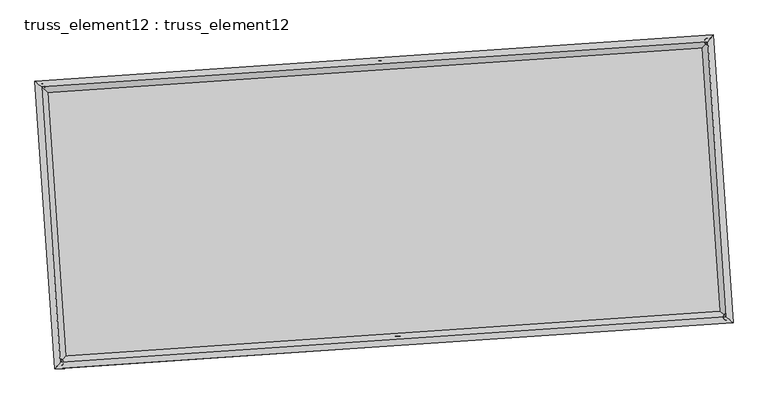
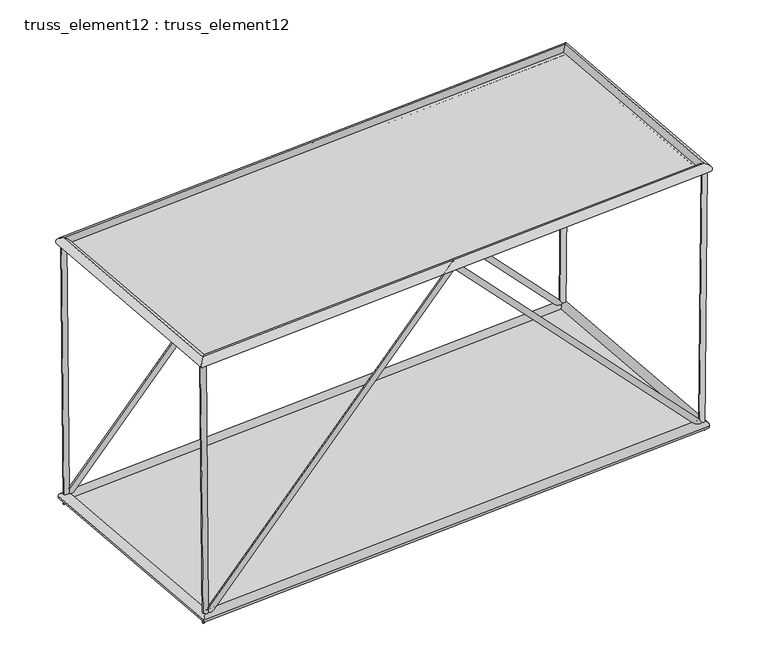
"""IFC4 building model written with IfcOpenShell, lengths in millimetres: plate geometry, truss_element12 : truss_element12."""

from ifc_helpers import new_model, si_unit, frame, origin, origin_with_axes, place, context, project, spatial, polyline, circle_curve, ellipse_curve, outline, extrude, source, transform, mapped, element, save
from ifc_brep_helpers import plane_surface, cylinder_surface, advanced_brep


def truss_element12_truss_element12_3d995396(model_context):
    return source(origin(), model_context, "Body", "SolidModel", [
        advanced_brep(
        [(-3712.6408018, 2272.9715483, 5000.2484753), (-3811.7396164, 2259.6106092, 4999.2944024), (-3666.1125982, 2276.1441296, 122.9707334), (-3762.8742846, 2262.9425505, -122.9707334), (1064.1401196, 2598.6820811, 5071.8896086), (1064.5820396, 2592.1084463, 4927.6451952), (5793.5718475, 2921.1640524, 122.9648431), (5891.1891295, 2921.2164361, -122.9648431), (5840.9148394, 2924.392191, 5000.2487538), (5940.9098971, 2924.6067063, 4999.2779762)],
        [
            (0, 1, circle_curve(frame((-3762.1902091, 2266.2910788, 4999.7714389), z_axis=(-0.009539353531426898, -0.0006504522548332356, 0.9999542877782298), x_axis=(-0.13360948886072543, 0.9910338579689815, -0.0006299567385858392)), 50.0)),
            (1, 0, circle_curve(frame((-3762.1902091, 2266.2910788, 4999.7714389), z_axis=(-0.009539353531426898, -0.0006504522548332356, 0.9999542877782298), x_axis=(-0.13360948886072543, 0.9910338579689815, -0.0006299567385858392)), 50.0)),
            (0, 2),
            (2, 3, ellipse_curve(frame((-3714.4934414, 2269.54334, 0.0), z_axis=(-0.9275444537546121, -0.06324573037496291, 0.368322228352289), x_axis=(0.3674689716323781, 0.02505631229527238, 0.9296981962452139)), 132.5575344, 50.0)),
            (3, 1),
            (3, 2, ellipse_curve(frame((-3714.4934414, 2269.54334, 0.0), z_axis=(-0.9275444537546121, -0.06324573037496291, 0.368322228352289), x_axis=(0.3674689716323781, 0.02505631229527238, 0.9296981962452139)), 132.5575344, 50.0)),
            (2, 4),
            (4, 5, ellipse_curve(frame((1064.3610796, 2595.3952637, 4999.7674019), z_axis=(-0.9976833951243609, -0.06802823816388774, 4.365141464773057e-05), x_axis=(-4.355029160929896e-05, -2.969528831717673e-06, -0.9999999990472769)), 72.279252, 50.0)),
            (5, 3),
            (5, 4, ellipse_curve(frame((1064.3610796, 2595.3952637, 4999.7674019), z_axis=(-0.9976833951243609, -0.06802823816388774, 4.365141464773057e-05), x_axis=(-4.355029160929896e-05, -2.969528831717673e-06, -0.9999999990472769)), 72.279252, 50.0)),
            (4, 6),
            (6, 7, ellipse_curve(frame((5842.3804885, 2921.1902443, 0.0), z_axis=(-0.9275912472386779, -0.06324892104476065, -0.36820381860169205), x_axis=(-0.36735083619027376, -0.02504825708855556, 0.9297450983829559)), 132.5444982, 50.0)),
            (7, 5),
            (7, 6, ellipse_curve(frame((5842.3804885, 2921.1902443, 0.0), z_axis=(-0.9275912472386779, -0.06324892104476065, -0.36820381860169205), x_axis=(-0.36735083619027376, -0.02504825708855556, 0.9297450983829559)), 132.5444982, 50.0)),
            (8, 9, circle_curve(frame((5890.9123683, 2924.4994486, 4999.763365), z_axis=(0.009706375954598431, 0.0006618408789518583, 0.999952672996317), x_axis=(-0.0021514761027001668, 0.999997480140261, -0.0006409865112665113)), 50.0)),
            (9, 8, circle_curve(frame((5890.9123683, 2924.4994486, 4999.763365), z_axis=(0.009706375954598431, 0.0006618408789518583, 0.999952672996317), x_axis=(-0.0021514761027001668, 0.999997480140261, -0.0006409865112665113)), 50.0)),
            (6, 8),
            (9, 7),
        ],
        [
            plane_surface(frame((-3762.1902091, 2316.2910682, 4999.803963), z_axis=(-0.009539353531428214, -0.0006504522548355754, 0.9999542877782297), x_axis=(0.9999544993319458, -6.205176354079358e-06, 0.009539351513250697))),
            cylinder_surface(frame((-3762.1902091, 2266.2910788, 4999.7714389), z_axis=(-0.009539353531426898, -0.0006504522548332356, 0.9999542877782298), x_axis=(-0.13360948886072543, 0.9910338579689815, -0.0006299567385858392)), 50.0),
            cylinder_surface(frame((-3714.4934414, 2269.54334, 0.0), z_axis=(-0.6901903584114236, -0.0470614568808942, -0.7220958997475049), x_axis=(-0.020415575362847597, 0.998752120640053, -0.04557856732721049)), 50.0),
            cylinder_surface(frame((1064.3610796, 2595.3952637, 4999.7674019), z_axis=(-0.6901274608072349, -0.047057168132365004, 0.7221562924790736), x_axis=(-0.11534925319653908, 0.9922789540252682, -0.04557441371559841)), 50.0),
            plane_surface(frame((5890.9123683, 2874.4994596, 4999.7964586), z_axis=(0.009706375954601498, 0.0006618408789477092, 0.9999526729963171), x_axis=(0.9999528920233334, -6.42437903231041e-06, -0.009706373828542777))),
            cylinder_surface(frame((5842.3804885, 2921.1902443, 0.0), z_axis=(-0.00970637595459843, -0.0006618408789518581, -0.9999526729963167), x_axis=(-0.0021514761027001668, 0.999997480140261, -0.0006409865112665113)), 50.0),
        ],
        [
            (0, [[1, 2]]),
            (1, [[-1, 3, 4, 5]]),
            (1, [[-2, -5, 6, -3]]),
            (2, [[-4, 7, 8, 9]]),
            (2, [[-6, -9, 10, -7]]),
            (3, [[-8, 11, 12, 13]]),
            (3, [[-10, -13, 14, -11]]),
            (4, [[15, 16]]),
            (5, [[-12, 17, -16, 18]]),
            (5, [[-14, -18, -15, -17]]),
        ],
    ),
        advanced_brep(
        [(-3440.5278489, -1717.762036, 5000.2484753), (-3539.6266635, -1731.1229751, 4999.2944024), (-3393.9996453, -1714.5894547, 122.9707334), (-3490.7613317, -1727.7910338, -122.9707334), (1336.2530725, -1392.0515032, 5071.8896086), (1336.6949926, -1398.625138, 4927.6451952), (6065.6848004, -1069.5695319, 122.9648431), (6163.3020824, -1069.5171482, -122.9648431), (6113.0277923, -1066.3413933, 5000.2487538), (6213.0228501, -1066.126878, 4999.2779762)],
        [
            (0, 1, circle_curve(frame((-3490.0772562, -1724.4425055, 4999.7714389), z_axis=(-0.009539353531426684, -0.0006504522548331923, 0.9999542877782298), x_axis=(-0.1336094888607254, 0.9910338579689815, -0.0006299567385858533)), 50.0)),
            (1, 0, circle_curve(frame((-3490.0772562, -1724.4425055, 4999.7714389), z_axis=(-0.009539353531426684, -0.0006504522548331923, 0.9999542877782298), x_axis=(-0.1336094888607254, 0.9910338579689815, -0.0006299567385858533)), 50.0)),
            (0, 2),
            (2, 3, ellipse_curve(frame((-3442.3804885, -1721.1902443, 0.0), z_axis=(-0.9275444537546114, -0.06324573037496278, 0.3683222283522907), x_axis=(0.36746897163237974, 0.025056312295272495, 0.9296981962452131)), 132.5575344, 50.0)),
            (3, 1),
            (3, 2, ellipse_curve(frame((-3442.3804885, -1721.1902443, 0.0), z_axis=(-0.9275444537546114, -0.06324573037496278, 0.3683222283522907), x_axis=(0.36746897163237974, 0.025056312295272495, 0.9296981962452131)), 132.5575344, 50.0)),
            (2, 4),
            (4, 5, ellipse_curve(frame((1336.4740325, -1395.3383206, 4999.7674019), z_axis=(-0.9976833951243609, -0.06802823816388762, 4.365141464997738e-05), x_axis=(-4.355029161160519e-05, -2.9695288319579026e-06, -0.9999999990472771)), 72.279252, 50.0)),
            (5, 3),
            (5, 4, ellipse_curve(frame((1336.4740325, -1395.3383206, 4999.7674019), z_axis=(-0.9976833951243609, -0.06802823816388762, 4.365141464997738e-05), x_axis=(-4.355029161160519e-05, -2.9695288319579026e-06, -0.9999999990472771)), 72.279252, 50.0)),
            (4, 6),
            (6, 7, ellipse_curve(frame((6114.4934414, -1069.54334, 0.0), z_axis=(-0.927591247238678, -0.06324892104476053, -0.3682038186016914), x_axis=(-0.3673508361902732, -0.025048257088555438, 0.929745098382956)), 132.5444982, 50.0)),
            (7, 5),
            (7, 6, ellipse_curve(frame((6114.4934414, -1069.54334, 0.0), z_axis=(-0.927591247238678, -0.06324892104476053, -0.3682038186016914), x_axis=(-0.3673508361902732, -0.025048257088555438, 0.929745098382956)), 132.5444982, 50.0)),
            (8, 9, circle_curve(frame((6163.0253212, -1066.2341357, 4999.763365), z_axis=(0.009706375954599215, 0.0006618408789519453, 0.999952672996317), x_axis=(-0.002151476102700382, 0.9999974801402611, -0.0006409865112665946)), 50.0)),
            (9, 8, circle_curve(frame((6163.0253212, -1066.2341357, 4999.763365), z_axis=(0.009706375954599215, 0.0006618408789519453, 0.999952672996317), x_axis=(-0.002151476102700382, 0.9999974801402611, -0.0006409865112665946)), 50.0)),
            (6, 8),
            (9, 7),
        ],
        [
            plane_surface(frame((-3490.0772562, -1674.4425161, 4999.803963), z_axis=(-0.009539353531428214, -0.0006504522548355842, 0.9999542877782297), x_axis=(0.9999544993319458, -6.205176354079358e-06, 0.009539351513250697))),
            cylinder_surface(frame((-3490.0772562, -1724.4425055, 4999.7714389), z_axis=(-0.009539353531426684, -0.0006504522548331923, 0.9999542877782298), x_axis=(-0.1336094888607254, 0.9910338579689815, -0.0006299567385858533)), 50.0),
            cylinder_surface(frame((-3442.3804885, -1721.1902443, 0.0), z_axis=(-0.6901903584114265, -0.047061456880894366, -0.7220958997475021), x_axis=(-0.020415575362847802, 0.998752120640053, -0.04557856732721061)), 50.0),
            cylinder_surface(frame((1336.4740325, -1395.3383206, 4999.7674019), z_axis=(-0.6901274608072342, -0.047057168132364824, 0.722156292479074), x_axis=(-0.1153492531965389, 0.9922789540252682, -0.04557441371559837)), 50.0),
            plane_surface(frame((6163.0253212, -1116.2341247, 4999.7964586), z_axis=(0.009706375954601498, 0.0006618408789477163, 0.9999526729963171), x_axis=(0.9999528920233334, -6.424379032754499e-06, -0.009706373828542777))),
            cylinder_surface(frame((6114.4934414, -1069.54334, 0.0), z_axis=(-0.009706375954599215, -0.0006618408789519453, -0.999952672996317), x_axis=(-0.002151476102700382, 0.9999974801402611, -0.0006409865112665946)), 50.0),
        ],
        [
            (0, [[1, 2]]),
            (1, [[-1, 3, 4, 5]]),
            (1, [[-2, -5, 6, -3]]),
            (2, [[-4, 7, 8, 9]]),
            (2, [[-6, -9, 10, -7]]),
            (3, [[-8, 11, 12, 13]]),
            (3, [[-10, -13, 14, -11]]),
            (4, [[15, 16]]),
            (5, [[-12, 17, -16, 18]]),
            (5, [[-14, -18, -15, -17]]),
        ],
    ),
        advanced_brep(
        [(-3490.0793814, -1724.444861, 4909.7714389), (-3490.075131, -1724.4401501, 5089.7714389), (-3762.1877838, 2266.2890336, 5089.7714389), (-3762.1926343, 2266.2931239, 4909.7714389), (5890.9103929, 2924.4971034, 5089.763365), (5890.9143436, 2924.5017939, 4909.763365), (6163.0230458, -1066.2320803, 5089.763365), (6163.0275966, -1066.236191, 4909.763365)],
        [
            (0, 1, ellipse_curve(frame((-3490.0772562, -1724.4425055, 4999.7714389), z_axis=(-0.7535719234052061, 0.6573654662781049, 5.900579994198024e-07), x_axis=(-0.6573654662778425, -0.7535719234054348, 5.900580116710992e-07)), 127.2792206, 90.0)),
            (1, 2),
            (2, 3, ellipse_curve(frame((-3762.1902091, 2266.2910788, 4999.7714389), z_axis=(-0.6573654662778421, -0.7535719234054352, 5.900580091387355e-07), x_axis=(0.7535719234052064, -0.6573654662781044, -5.900579968874395e-07)), 127.2792206, 90.0)),
            (3, 0),
            (1, 0, ellipse_curve(frame((-3490.0772562, -1724.4425055, 4999.7714389), z_axis=(-0.7535719234052061, 0.6573654662781049, 5.900579994198024e-07), x_axis=(-0.6573654662778425, -0.7535719234054348, 5.900580116710992e-07)), 127.2792206, 90.0)),
            (3, 2, ellipse_curve(frame((-3762.1902091, 2266.2910788, 4999.7714389), z_axis=(-0.6573654662778421, -0.7535719234054352, 5.900580091387355e-07), x_axis=(0.7535719234052064, -0.6573654662781044, -5.900579968874395e-07)), 127.2792206, 90.0)),
            (2, 4),
            (4, 5, ellipse_curve(frame((5890.9123683, 2924.4994486, 4999.763365), z_axis=(-0.753571923405209, 0.6573654662781013, 5.90058003013114e-07), x_axis=(-0.6573654662778391, -0.7535719234054377, 5.900580030130607e-07)), 127.2792206, 90.0)),
            (5, 3),
            (5, 4, ellipse_curve(frame((5890.9123683, 2924.4994486, 4999.763365), z_axis=(-0.753571923405209, 0.6573654662781013, 5.90058003013114e-07), x_axis=(-0.6573654662778391, -0.7535719234054377, 5.900580030130607e-07)), 127.2792206, 90.0)),
            (4, 6),
            (6, 7, ellipse_curve(frame((6163.0253212, -1066.2341357, 4999.763365), z_axis=(0.6573654662778391, 0.7535719234054377, -5.900580055454242e-07), x_axis=(-0.7535719234052087, 0.6573654662781017, 5.900580055454772e-07)), 127.2792206, 90.0)),
            (7, 5),
            (7, 6, ellipse_curve(frame((6163.0253212, -1066.2341357, 4999.763365), z_axis=(0.6573654662778391, 0.7535719234054377, -5.900580055454242e-07), x_axis=(-0.7535719234052087, 0.6573654662781017, 5.900580055454772e-07)), 127.2792206, 90.0)),
            (6, 1),
            (0, 7),
        ],
        [
            cylinder_surface(frame((-3490.0772562, -1724.4425055, 4999.7714389), z_axis=(0.06802823822868706, -0.9976833960748777, 0.0), x_axis=(-0.9976833957545878, -0.06802823820684771, 2.53390411256576e-05)), 90.0),
            cylinder_surface(frame((-3762.1902091, 2266.2910788, 4999.7714389), z_axis=(-0.9976833960745297, -0.06802823822867328, 8.344680304478929e-07), x_axis=(-0.06802823818787146, 0.9976833957767265, 2.450457308679736e-05)), 90.0),
            cylinder_surface(frame((5890.9123683, 2924.4994486, 4999.763365), z_axis=(-0.06802823822869537, 0.9976833960748771, 0.0), x_axis=(0.9976833957953891, 0.06802823820963814, 2.3670105056600042e-05)), 90.0),
            cylinder_surface(frame((6163.0253212, -1066.2341357, 4999.763365), z_axis=(0.9976833960745297, 0.06802823822867272, -8.344680340291955e-07), x_axis=(0.06802823822867272, -0.9976833957739445, 2.450457309037874e-05)), 90.0),
        ],
        [
            (0, [[1, 2, 3, 4]]),
            (0, [[5, -4, 6, -2]]),
            (1, [[-3, 7, 8, 9]]),
            (1, [[-6, -9, 10, -7]]),
            (2, [[-8, 11, 12, 13]]),
            (2, [[-10, -13, 14, -11]]),
            (3, [[-12, 15, -1, 16]]),
            (3, [[-14, -16, -5, -15]]),
        ],
    ),
        advanced_brep(
        [(-3358.7115243, -1625.2761972, 0.0), (-3526.0494527, -1817.1042913, 0.0), (-3810.4074885, 2353.2123043, 0.0), (-3618.5793943, 2185.8743758, 0.0), (5926.0494527, 3017.1042913, 0.0), (5758.7115243, 2825.2761972, 0.0), (6210.4074885, -1153.2123043, 0.0), (6018.5793943, -985.8743758, 0.0)],
        [
            (0, 1, ellipse_curve(frame((-3442.3804885, -1721.1902443, 0.0), z_axis=(-0.7535719234054536, 0.6573654662780856, 0.0), x_axis=(-0.6573654662780855, -0.7535719234054539, 0.0)), 127.2792206, 90.0)),
            (1, 2),
            (2, 3, ellipse_curve(frame((-3714.4934414, 2269.54334, 0.0), z_axis=(-0.6573654662780855, -0.7535719234054539, 0.0), x_axis=(0.7535719234054538, -0.6573654662780856, 0.0)), 127.2792206, 90.0)),
            (3, 0),
            (1, 0, ellipse_curve(frame((-3442.3804885, -1721.1902443, 0.0), z_axis=(-0.7535719234054536, 0.6573654662780856, 0.0), x_axis=(-0.6573654662780855, -0.7535719234054539, 0.0)), 127.2792206, 90.0)),
            (3, 2, ellipse_curve(frame((-3714.4934414, 2269.54334, 0.0), z_axis=(-0.6573654662780855, -0.7535719234054539, 0.0), x_axis=(0.7535719234054538, -0.6573654662780856, 0.0)), 127.2792206, 90.0)),
            (2, 4),
            (4, 5, ellipse_curve(frame((5842.3804885, 2921.1902443, 0.0), z_axis=(-0.7535719234054568, 0.6573654662780822, 0.0), x_axis=(-0.657365466278082, -0.7535719234054568, 0.0)), 127.2792206, 90.0)),
            (5, 3),
            (5, 4, ellipse_curve(frame((5842.3804885, 2921.1902443, 0.0), z_axis=(-0.7535719234054568, 0.6573654662780822, 0.0), x_axis=(-0.657365466278082, -0.7535719234054568, 0.0)), 127.2792206, 90.0)),
            (4, 6),
            (6, 7, ellipse_curve(frame((6114.4934414, -1069.54334, 0.0), z_axis=(0.6573654662780823, 0.7535719234054566, 0.0), x_axis=(-0.7535719234054565, 0.6573654662780822, 0.0)), 127.2792206, 90.0)),
            (7, 5),
            (7, 6, ellipse_curve(frame((6114.4934414, -1069.54334, 0.0), z_axis=(0.6573654662780823, 0.7535719234054566, 0.0), x_axis=(-0.7535719234054565, 0.6573654662780822, 0.0)), 127.2792206, 90.0)),
            (6, 1),
            (0, 7),
        ],
        [
            cylinder_surface(frame((-3442.3804885, -1721.1902443, 0.0), z_axis=(0.06802823822869013, -0.9976833960748773, 0.0), x_axis=(-0.9976833960748773, -0.06802823822869013, 0.0)), 90.0),
            cylinder_surface(frame((-3714.4934414, 2269.54334, 0.0), z_axis=(-0.9976833960748767, -0.06802823822869991, 0.0), x_axis=(-0.06802823822869991, 0.9976833960748767, 0.0)), 90.0),
            cylinder_surface(frame((5842.3804885, 2921.1902443, 0.0), z_axis=(-0.06802823822869869, 0.9976833960748768, 0.0), x_axis=(0.9976833960748768, 0.06802823822869869, 0.0)), 90.0),
            cylinder_surface(frame((6114.4934414, -1069.54334, 0.0), z_axis=(0.9976833960748768, 0.06802823822869974, 0.0), x_axis=(0.06802823822869974, -0.9976833960748768, 0.0)), 90.0),
        ],
        [
            (0, [[1, 2, 3, 4]]),
            (0, [[5, -4, 6, -2]]),
            (1, [[-3, 7, 8, 9]]),
            (1, [[-6, -9, 10, -7]]),
            (2, [[-8, 11, 12, 13]]),
            (2, [[-10, -13, 14, -11]]),
            (3, [[-12, 15, -1, 16]]),
            (3, [[-14, -16, -5, -15]]),
        ],
    ),
        extrude(outline(polyline([(-3442.3804885, -1721.1902443), (-3714.4934414, 2269.54334), (5842.3804885, 2921.1902443), (6114.4934414, -1069.54334), (-3442.3804885, -1721.1902443)])), origin_with_axes(), (0.0, 0.0, 1.0), 20.0),
        extrude(outline(polyline([(-2000.0, 4837.758459), (2000.0, 4837.758459), (1999.9999999, -4837.7584589), (-2000.0000001, -4837.7584589), (-2000.0, 4837.758459)])), frame((1200.4175561, 600.0284716, 4999.7674019), z_axis=(8.32534897943804e-07, 5.67673986124007e-08, 0.999999999999652), x_axis=(-0.06802823822868996, 0.9976833960748774, 0.0)), (0.0, 0.0, 1.0), 20.0),
    ])


if __name__ == "__main__":
    model = new_model("IFC4")
    model_context = context("Model", 3, world=origin())
    ifc_project = project(units=[si_unit("LENGTHUNIT", "METRE", prefix="MILLI")], contexts=[model_context])
    site = spatial("IfcSite", under=ifc_project)
    building = spatial("IfcBuilding", under=site)
    placement = place(None, origin())
    truss_element12_truss_element12_shape = truss_element12_truss_element12_3d995396(model_context)
    element("IfcPlate", 1, ObjectType="truss_element12 : truss_element12", at=placement, inside=building, context=model_context, shape_type="MappedRepresentation", body=[
        mapped(truss_element12_truss_element12_shape, transform((0.0, 0.0, 0.0), x_axis=(1.0, 0.0, 0.0), y_axis=(0.0, 1.0, 0.0), z_axis=(0.0, 0.0, 1.0))),
    ])
    save(model, "model.ifc")

# Revit data of these elements
# Type "truss_element12 : truss_element12"
#   steellbar1 = 90 mm
#   steelbar2 = 50 mm
#   offset1 = 5000 mm
#   M = Default Roof
# Element 1 (IfcPlate, "truss_element12 : truss_element12")
#   Materials on its faces: "Default Roof"
# Materials
#   "Default Roof": class "Miscellaneous", colour RGB 0 127 0, transparency 0, Comments = "Rendering appearance not upgraded Rendering appearance not upgraded ", Cost = 0
